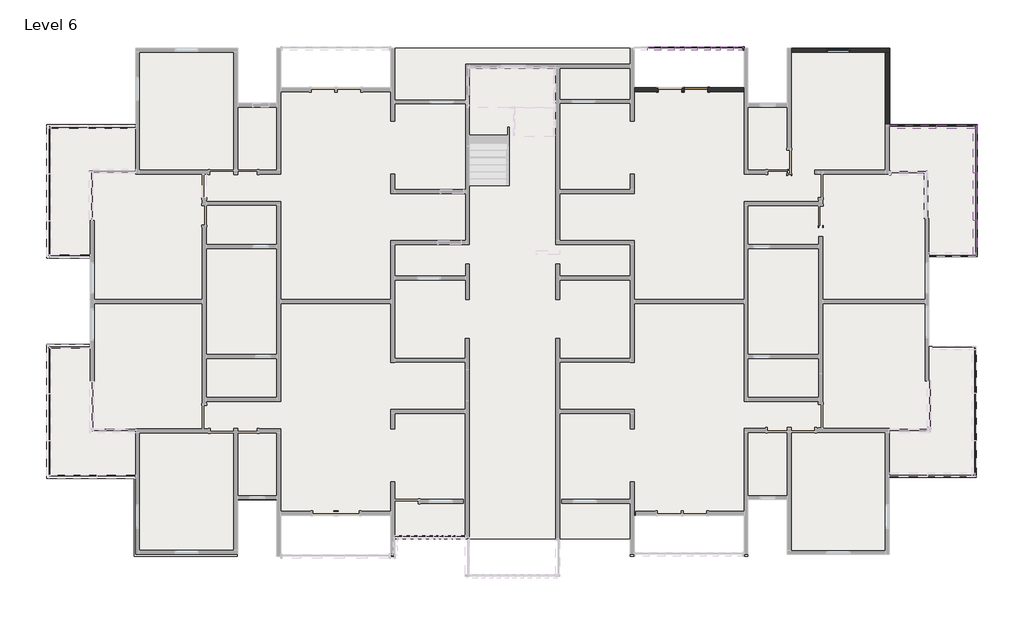
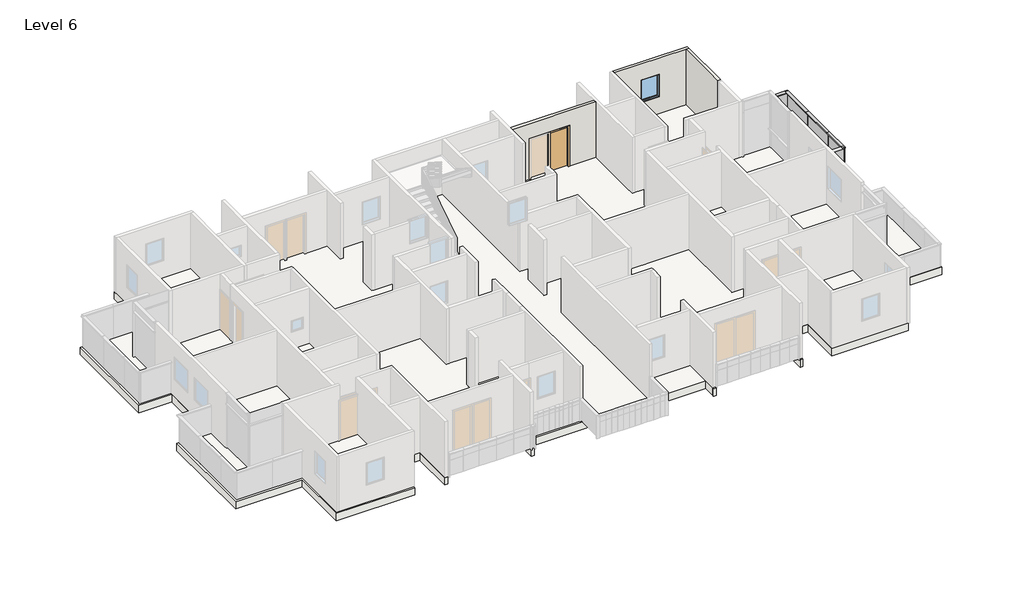
# One storey, part 5 of 7: 14 members, 13 plates, 3 walls, 1 door, 1 slab, 1 window.
"""IFC4 building model written with IfcOpenShell, lengths in millimetres."""

import ifcopenshell
import ifcopenshell.guid

model = None  # the IFC model being written
_history = None  # IfcOwnerHistory: only IFC2X3 demands one
_inside = {}  # id of a spatial element -> (the spatial element, [elements in it])
_under = {}  # id of a project, library or spatial element -> (it, [spatial elements below it])
_declared = {}  # id of a project -> (the project, [libraries it declares])
_typed = {}  # id of a type object -> (the type object, [elements of that type])
_made_of = {}  # id of a material, layer set ... -> (it, [elements and type objects made of it])


def new_model(schema):
    """Start an empty IFC model of exactly this schema.

    Asked for "IFC4X3", IfcOpenShell would pick the latest addendum, in which some entities
    have other attributes; the version numbers below select the first issue.
    IFC2X3 requires an IfcOwnerHistory on every rooted entity: one is made here for all.
    """
    global model, _history
    if schema == "IFC4X3":
        model = ifcopenshell.file(schema_version=(4, 3, 0, 0))
    else:
        model = ifcopenshell.file(schema=schema)
    _inside.clear()
    _under.clear()
    _declared.clear()
    _typed.clear()
    _made_of.clear()
    _history = None
    if model.schema == "IFC2X3":
        org = make("IfcOrganization", Name="unknown")
        user = make(
            "IfcPersonAndOrganization",
            ThePerson=make("IfcPerson", FamilyName="unknown"),
            TheOrganization=org,
        )
        app = make(
            "IfcApplication",
            ApplicationDeveloper=org,
            Version="unknown",
            ApplicationFullName="unknown",
            ApplicationIdentifier="unknown",
        )
        _history = make(
            "IfcOwnerHistory",
            OwningUser=user,
            OwningApplication=app,
            ChangeAction="ADDED",
            CreationDate=0,
        )
    return model


def make(cls, **values):
    """One entity of the class cls with the attributes given. An attribute that is None is left unset."""
    return model.create_entity(
        cls, **{name: value for name, value in values.items() if value is not None}
    )


def rooted(cls, **values):
    """An entity with a GlobalId (a new one), such as an element, a storey or a relation."""
    return make(cls, GlobalId=ifcopenshell.guid.new(), OwnerHistory=_history, **values)


def si_unit(unit_type, name, prefix=None):
    """IfcSIUnit, for example si_unit("LENGTHUNIT", "METRE", prefix="MILLI")."""
    return make("IfcSIUnit", UnitType=unit_type, Prefix=prefix, Name=name)


def assignment(units):
    """IfcUnitAssignment: the units of a project."""
    return None if units is None else make("IfcUnitAssignment", Units=units)


def point(xyz):
    """IfcCartesianPoint."""
    return None if xyz is None else make("IfcCartesianPoint", Coordinates=xyz)


def direction(xyz):
    """IfcDirection."""
    return None if xyz is None else make("IfcDirection", DirectionRatios=xyz)


def frame(location, z_axis=None, x_axis=None):
    """IfcAxis2Placement3D, a coordinate frame: its origin and axes. An axis left out is left unset."""
    return make(
        "IfcAxis2Placement3D",
        Location=point(location),
        Axis=direction(z_axis),
        RefDirection=direction(x_axis),
    )


def origin():
    """The frame at (0, 0, 0) with its axes left unset."""
    return frame((0.0, 0.0, 0.0))


def origin_with_axes():
    """The frame at (0, 0, 0) with the z axis (0, 0, 1) and the x axis (1, 0, 0) written out."""
    return frame((0.0, 0.0, 0.0), z_axis=(0.0, 0.0, 1.0), x_axis=(1.0, 0.0, 0.0))


def place(relative_to, where):
    """IfcLocalPlacement: puts the frame where relative to a parent placement (None: the world)."""
    return make(
        "IfcLocalPlacement", PlacementRelTo=relative_to, RelativePlacement=where
    )


def context(
    kind, dimensions, precision=None, world=None, true_north=None, identifier=None
):
    """IfcGeometricRepresentationContext, for example the 3D "Model" context."""
    return make(
        "IfcGeometricRepresentationContext",
        ContextIdentifier=identifier,
        ContextType=kind,
        CoordinateSpaceDimension=dimensions,
        Precision=precision,
        WorldCoordinateSystem=world,
        TrueNorth=true_north,
    )


def project(units=None, contexts=None):
    """IfcProject with its units and contexts."""
    return rooted(
        "IfcProject",
        Name="project",
        RepresentationContexts=contexts,
        UnitsInContext=assignment(units),
    )


def spatial(cls, under=None, at=None, **own):
    """A site, building, storey or space (cls), placed at a placement, below another one or the project."""
    s = rooted(cls, ObjectPlacement=at, **own)
    if under is not None:
        _under.setdefault(under.id(), (under, []))[1].append(s)
    return s


def polyline(points):
    """IfcPolyline through the points."""
    return make("IfcPolyline", Points=[point(p) for p in points])


def outline(outer, holes=None, kind="AREA"):
    """IfcArbitraryClosedProfileDef: a profile drawn as a closed curve; with holes, ...WithVoids."""
    if holes is None:
        return make("IfcArbitraryClosedProfileDef", ProfileType=kind, OuterCurve=outer)
    return make(
        "IfcArbitraryProfileDefWithVoids",
        ProfileType=kind,
        OuterCurve=outer,
        InnerCurves=holes,
    )


def extrude(swept, where, along, depth):
    """IfcExtrudedAreaSolid: the profile swept, set in the frame where, extruded along a direction by depth."""
    return make(
        "IfcExtrudedAreaSolid",
        SweptArea=swept,
        Position=where,
        ExtrudedDirection=direction(along),
        Depth=depth,
    )


def faces_of(points, faces, orient=None, outer=None):
    """IfcFace entities. A face is a list of loops; a loop is a list of indices into points, from 0.

    orient and outer hold one flag for each loop. By default every Orientation is true, the
    first loop of a face is its IfcFaceOuterBound and the others are IfcFaceBound.
    """
    made = []
    for i, loops in enumerate(faces):
        bounds = []
        for j, loop in enumerate(loops):
            is_outer = j == 0 if outer is None else outer[i][j]
            bounds.append(
                make(
                    "IfcFaceOuterBound" if is_outer else "IfcFaceBound",
                    Bound=make("IfcPolyLoop", Polygon=[points[k] for k in loop]),
                    Orientation=True if orient is None else orient[i][j],
                )
            )
        made.append(make("IfcFace", Bounds=bounds))
    return made


def faceted_brep(points, faces, orient=None, outer=None, voids=None):
    """IfcFacetedBrep: a solid bounded by flat faces; with voids (closed shells), ...WithVoids."""
    shared = [point(p) for p in points]
    hull = make("IfcClosedShell", CfsFaces=faces_of(shared, faces, orient, outer))
    if voids is None:
        return make("IfcFacetedBrep", Outer=hull)
    return make(
        "IfcFacetedBrepWithVoids",
        Outer=hull,
        Voids=[
            make(cls, CfsFaces=faces_of(shared, fs, o, b)) for cls, fs, o, b in voids
        ],
    )


def shape(context_of_items, identifier, shape_type, items):
    """IfcShapeRepresentation: the items that make up one representation, for example the "Body"."""
    return make(
        "IfcShapeRepresentation",
        ContextOfItems=context_of_items,
        RepresentationIdentifier=identifier,
        RepresentationType=shape_type,
        Items=items,
    )


def source(mapping_origin, context_of_items, identifier, shape_type, items):
    """IfcRepresentationMap: a shape defined once, which mapped items show again and again."""
    return make(
        "IfcRepresentationMap",
        MappingOrigin=mapping_origin,
        MappedRepresentation=shape(context_of_items, identifier, shape_type, items),
    )


def transform(
    local_origin,
    x_axis=None,
    y_axis=None,
    z_axis=None,
    scale=None,
    scale2=None,
    scale3=None,
    uniform=True,
):
    """IfcCartesianTransformationOperator3D, or its non-uniform kind. x_axis, y_axis, z_axis: its Axis1, 2, 3."""
    if uniform:
        return make(
            "IfcCartesianTransformationOperator3D",
            Axis1=direction(x_axis),
            Axis2=direction(y_axis),
            LocalOrigin=point(local_origin),
            Scale=scale,
            Axis3=direction(z_axis),
        )
    return make(
        "IfcCartesianTransformationOperator3DnonUniform",
        Axis1=direction(x_axis),
        Axis2=direction(y_axis),
        LocalOrigin=point(local_origin),
        Scale=scale,
        Axis3=direction(z_axis),
        Scale2=scale2,
        Scale3=scale3,
    )


def mapped(mapping_source, mapping_target):
    """IfcMappedItem: shows the shape of a source again, moved by a transform."""
    return make(
        "IfcMappedItem", MappingSource=mapping_source, MappingTarget=mapping_target
    )


def made_of(thing, what):
    """Note that an element or type object is made of a material, layer set ...; save() writes the relation."""
    if what is not None:
        _made_of.setdefault(what.id(), (what, []))[1].append(thing)
    return thing


def element(
    cls,
    number,
    at=None,
    inside=None,
    cuts=None,
    type_object=None,
    material=None,
    context=None,
    identifier="Body",
    shape_type=None,
    held_by="IfcProductDefinitionShape",
    body=None,
    shapes=None,
    **own,
):
    """One element of the class cls, such as IfcWall. Its Tag is "e" and its number.

    at: its placement. inside: the storey or other place that contains it. cuts: it is an
    opening in that element (IfcRelVoidsElement). A single representation is given by context,
    identifier, shape_type and body (its items); several are given by shapes. held_by: the class
    of the entity that holds the representations. save() writes the other relations.
    """
    e = rooted(cls, Tag="e%d" % number, ObjectPlacement=at, **own)
    if body is not None:
        shapes = [shape(context, identifier, shape_type, body)]
    if shapes is not None:
        e.Representation = make(held_by, Representations=shapes)
    if inside is not None:
        _inside.setdefault(inside.id(), (inside, []))[1].append(e)
    if cuts is not None:
        rooted(
            "IfcRelVoidsElement", RelatingBuildingElement=cuts, RelatedOpeningElement=e
        )
    if type_object is not None:
        _typed.setdefault(type_object.id(), (type_object, []))[1].append(e)
    return made_of(e, material)


def aggregate(whole, parts):
    """IfcRelAggregates: a whole, such as a stair, and the parts it consists of."""
    return rooted("IfcRelAggregates", RelatingObject=whole, RelatedObjects=parts)


def save(model, path):
    """Write the relations noted so far, then the file.

    IfcRelAggregates (storeys below a building ...), IfcRelContainedInSpatialStructure (elements
    in a storey), IfcRelDefinesByType, IfcRelAssociatesMaterial and IfcRelDeclares: one each for
    every whole, place, type object, material and project.
    """
    for whole, parts in _under.values():
        aggregate(whole, parts)
    for where, things in _inside.values():
        rooted(
            "IfcRelContainedInSpatialStructure",
            RelatedElements=things,
            RelatingStructure=where,
        )
    for kind, things in _typed.values():
        rooted("IfcRelDefinesByType", RelatedObjects=things, RelatingType=kind)
    for what, things in _made_of.values():
        rooted("IfcRelAssociatesMaterial", RelatedObjects=things, RelatingMaterial=what)
    for by, libraries in _declared.values():
        rooted("IfcRelDeclares", RelatingContext=by, RelatedDefinitions=libraries)
    model.write(path)


def m_single_flush_0915_x_2134mm_138fd904(model_context):
    return source(origin(), model_context, "Body", "SweptSolid", [
        extrude(outline(polyline([(2210.0, -533.5), (0.0, -533.5), (0.0, -457.5), (2134.0, -457.5), (2134.0, 457.5), (0.0, 457.5), (0.0, 533.5), (2210.0, 533.5), (2210.0, -533.5)])), frame((0.0, 75.0, 0.0), z_axis=(0.0, 1.0, 0.0), x_axis=(0.0, 0.0, 1.0)), (0.0, 0.0, 1.0), 25.0),
        extrude(outline(polyline([(2210.0, 533.5), (2210.0, -533.5), (0.0, -533.5), (0.0, -457.5), (2134.0, -457.5), (2134.0, 457.5), (0.0, 457.5), (0.0, 533.5), (2210.0, 533.5)])), frame((0.0, -100.0, 0.0), z_axis=(0.0, 1.0, 0.0), x_axis=(0.0, 0.0, 1.0)), (0.0, 0.0, 1.0), 25.0),
        extrude(outline(polyline([(457.5, 24.0), (-457.5, 24.0), (-457.5, 75.0), (457.5, 75.0), (457.5, 24.0)])), origin_with_axes(), (0.0, 0.0, 1.0), 2134.0),
    ])


def rectangular_mullion_50mm_x_150mm_42770ee2(model_context):
    return source(origin(), model_context, "Body", "SweptSolid", [
        extrude(outline(polyline([(0.0, 75.0), (0.0, -75.0), (-50.0, -75.0), (-50.0, 75.0), (0.0, 75.0)])), frame((0.0, 0.0, -1830.0000003), z_axis=(0.0, 0.0, 1.0), x_axis=(1.0, 0.0, 0.0)), (0.0, 0.0, 1.0), 1830.0000003),
    ])


def rectangular_mullion_50mm_x_150mm_aaee7d48(model_context):
    return source(origin(), model_context, "Body", "SweptSolid", [
        extrude(outline(polyline([(0.0, 75.0), (0.0, -75.0), (-50.0, -75.0), (-50.0, 75.0), (0.0, 75.0)])), frame((0.0, 0.0, -1830.0), z_axis=(0.0, 0.0, 1.0), x_axis=(1.0, 0.0, 0.0)), (0.0, 0.0, 1.0), 1830.0),
    ])


def rectangular_mullion_50mm_x_150mm_efa02866(model_context):
    return source(origin(), model_context, "Body", "SweptSolid", [
        extrude(outline(polyline([(0.0, 75.0), (0.0, -75.0), (-50.0, -75.0), (-50.0, 75.0), (0.0, 75.0)])), frame((0.0, 0.0, -1399.9999997), z_axis=(0.0, 0.0, 1.0), x_axis=(1.0, 0.0, 0.0)), (0.0, 0.0, 1.0), 1399.9999997),
    ])


def rectangular_mullion_50mm_x_150mm_d9f1e9e9(model_context):
    return source(origin(), model_context, "Body", "SweptSolid", [
        extrude(outline(polyline([(0.0, 75.0), (0.0, -75.0), (-50.0, -75.0), (-50.0, 75.0), (0.0, 75.0)])), frame((0.0, 0.0, -1565.8160321), z_axis=(0.0, 0.0, 1.0), x_axis=(1.0, 0.0, 0.0)), (0.0, 0.0, 1.0), 1565.8160321),
    ])


def rectangular_mullion_50mm_x_150mm_729c0cfc(model_context):
    return source(origin(), model_context, "Body", "SweptSolid", [
        extrude(outline(polyline([(0.0, 75.0), (0.0, -75.0), (-50.0, -75.0), (-50.0, 75.0), (0.0, 75.0)])), frame((0.0, 0.0, -1250.0), z_axis=(0.0, 0.0, 1.0), x_axis=(1.0, 0.0, 0.0)), (0.0, 0.0, 1.0), 1250.0),
    ])


def rectangular_mullion_50mm_x_150mm_b3666dbd(model_context):
    return source(origin(), model_context, "Body", "SweptSolid", [
        extrude(outline(polyline([(0.0, 75.0), (0.0, -75.0), (-50.0, -75.0), (-50.0, 75.0), (0.0, 75.0)])), frame((0.0, 0.0, -500.0), z_axis=(0.0, 0.0, 1.0), x_axis=(1.0, 0.0, 0.0)), (0.0, 0.0, 1.0), 500.0),
    ])


def rectangular_mullion_50mm_x_150mm_e851a0b8(model_context):
    return source(origin(), model_context, "Body", "SweptSolid", [
        extrude(outline(polyline([(0.0, 75.0), (0.0, -75.0), (-50.0, -75.0), (-50.0, 75.0), (0.0, 75.0)])), frame((0.0, 0.0, -522.7272727), z_axis=(0.0, 0.0, 1.0), x_axis=(1.0, 0.0, 0.0)), (0.0, 0.0, 1.0), 522.7272727),
    ])


def rectangular_mullion_50mm_x_150mm_e11a3e7b(model_context):
    return source(origin(), model_context, "Body", "SweptSolid", [
        extrude(outline(polyline([(0.0, 75.0), (0.0, -75.0), (-50.0, -75.0), (-50.0, 75.0), (0.0, 75.0)])), frame((0.0, 0.0, -400.0), z_axis=(0.0, 0.0, 1.0), x_axis=(1.0, 0.0, 0.0)), (0.0, 0.0, 1.0), 400.0),
    ])


def rectangular_mullion_50mm_x_150mm_23485ade(model_context):
    return source(origin(), model_context, "Body", "SweptSolid", [
        extrude(outline(polyline([(0.0, 75.0), (0.0, -75.0), (-50.0, -75.0), (-50.0, 75.0), (0.0, 75.0)])), frame((0.0, 0.0, -350.0), z_axis=(0.0, 0.0, 1.0), x_axis=(1.0, 0.0, 0.0)), (0.0, 0.0, 1.0), 350.0),
    ])


def system_panel_glazed_09fbcc53(model_context):
    return source(origin(), model_context, "Body", "SweptSolid", [
        extrude(outline(polyline([(915.0000002, 24.5), (-915.0000002, 24.5), (-915.0000002, 49.5), (915.0000002, 49.5), (915.0000002, 24.5)])), origin_with_axes(), (0.0, 0.0, 1.0), 1200.0),
    ])


def system_panel_glazed_f4bbd109(model_context):
    return source(origin(), model_context, "Body", "SweptSolid", [
        extrude(outline(polyline([(910.8343113, 24.5), (-910.8343113, 24.5), (-910.8343113, 49.5), (910.8343113, 49.5), (910.8343113, 24.5)])), origin_with_axes(), (0.0, 0.0, 1.0), 1200.0),
    ])


def system_panel_glazed_42eec186(model_context):
    return source(origin(), model_context, "Body", "SweptSolid", [
        extrude(outline(polyline([(699.9999998, 24.5), (-699.9999998, 24.5), (-699.9999998, 49.5), (699.9999998, 49.5), (699.9999998, 24.5)])), origin_with_axes(), (0.0, 0.0, 1.0), 1200.0),
    ])


def system_panel_glazed_f2fc581d(model_context):
    return source(origin(), model_context, "Body", "SweptSolid", [
        extrude(outline(polyline([(782.9080161, 24.5), (-782.9080161, 24.5), (-782.9080161, 49.5), (782.9080161, 49.5), (782.9080161, 24.5)])), origin_with_axes(), (0.0, 0.0, 1.0), 1200.0),
    ])


def system_panel_glazed_346501af(model_context):
    return source(origin(), model_context, "Body", "SweptSolid", [
        extrude(outline(polyline([(250.0, 24.5), (-250.0, 24.5), (-250.0, 49.5), (250.0, 49.5), (250.0, 24.5)])), origin_with_axes(), (0.0, 0.0, 1.0), 1200.0),
    ])


def system_panel_glazed_5241e6d5(model_context):
    return source(origin(), model_context, "Body", "SweptSolid", [
        extrude(outline(polyline([(261.3636364, 24.5), (-261.3636364, 24.5), (-261.3636364, 49.5), (261.3636364, 49.5), (261.3636364, 24.5)])), origin_with_axes(), (0.0, 0.0, 1.0), 1200.0),
    ])


def system_panel_glazed_3e660766(model_context):
    return source(origin(), model_context, "Body", "SweptSolid", [
        extrude(outline(polyline([(200.0, 24.5), (-200.0, 24.5), (-200.0, 49.5), (200.0, 49.5), (200.0, 24.5)])), origin_with_axes(), (0.0, 0.0, 1.0), 1200.0),
    ])


def system_panel_glazed_b0a6d7cd(model_context):
    return source(origin(), model_context, "Body", "SweptSolid", [
        extrude(outline(polyline([(175.0, 24.5), (-175.0, 24.5), (-175.0, 49.5), (175.0, 49.5), (175.0, 24.5)])), origin_with_axes(), (0.0, 0.0, 1.0), 1200.0),
    ])


def m_fixed_0915_x_1220mm_873aa0e2(model_context):
    return source(origin(), model_context, "Body", "SweptSolid", [
        extrude(outline(polyline([(-394.5, 53.0), (394.5, 53.0), (394.5, 41.0), (-394.5, 41.0), (-394.5, 53.0)])), frame((0.0, 0.0, 978.0), z_axis=(0.0, 0.0, 1.0), x_axis=(1.0, 0.0, 0.0)), (0.0, 0.0, 1.0), 1094.0),
        extrude(outline(polyline([(2116.0, -438.5), (934.0, -438.5), (934.0, 438.5), (2116.0, 438.5), (2116.0, -438.5)]), holes=[polyline([(2072.0, -394.5), (2072.0, 394.5), (978.0, 394.5), (978.0, -394.5), (2072.0, -394.5)])]), frame((0.0, 25.0, 0.0), z_axis=(0.0, 1.0, 0.0), x_axis=(0.0, 0.0, 1.0)), (0.0, 0.0, 1.0), 44.0),
        extrude(outline(polyline([(2135.0, -457.5), (915.0, -457.5), (915.0, 457.5), (2135.0, 457.5), (2135.0, -457.5)]), holes=[polyline([(2116.0, -438.5), (2116.0, 438.5), (934.0, 438.5), (934.0, -438.5), (2116.0, -438.5)])]), frame((0.0, 25.0, 0.0), z_axis=(0.0, 1.0, 0.0), x_axis=(0.0, 0.0, 1.0)), (0.0, 0.0, 1.0), 63.0),
        extrude(outline(polyline([(2135.0, -457.5), (915.0, -457.5), (915.0, 457.5), (2135.0, 457.5), (2135.0, -457.5)]), holes=[polyline([(2103.0, -425.5), (2103.0, 425.5), (947.0, 425.5), (947.0, -425.5), (2103.0, -425.5)])]), frame((0.0, -62.0, 0.0), z_axis=(0.0, 1.0, 0.0), x_axis=(0.0, 0.0, 1.0)), (0.0, 0.0, 1.0), 87.0),
    ])


model = new_model("IFC4")

# Units and contexts
model_context = context("Model", 3, world=origin())
ifc_project = project(units=[si_unit("LENGTHUNIT", "METRE", prefix="MILLI")], contexts=[model_context])

# Site, building, storey
site = spatial("IfcSite", under=ifc_project)
building = spatial("IfcBuilding", under=site)
storey = spatial("IfcBuildingStorey", under=building, Name="Level 6", Elevation=15500.0)

# Door
placement = place(None, origin())
m_single_flush_0915_x_2134mm_shape = m_single_flush_0915_x_2134mm_138fd904(model_context)
element("IfcDoor", 1, ObjectType="M_Single-Flush : 0915 x 2134mm", at=placement, inside=storey, context=model_context, shape_type="MappedRepresentation", body=[
    mapped(m_single_flush_0915_x_2134mm_shape, transform((6794.6515415, 8016.5690894, 15500.0), x_axis=(1.0, 0.0, 0.0), y_axis=(0.0, 1.0, 0.0), z_axis=(0.0, 0.0, 1.0))),
])

# Members
rectangular_mullion_50mm_x_150mm_shape = rectangular_mullion_50mm_x_150mm_42770ee2(model_context)
element("IfcMember", 2, ObjectType="Rectangular Mullion : 50mm x 150mm", at=placement, inside=storey, context=model_context, shape_type="MappedRepresentation", body=[
    mapped(rectangular_mullion_50mm_x_150mm_shape, transform((17635.0130284, 4788.3418163, 16750.0), x_axis=(0.0, 0.0, 1.0), y_axis=(-1.0, 0.0, 0.0), z_axis=(0.0, -1.0, 0.0))),
])
element("IfcMember", 3, ObjectType="Rectangular Mullion : 50mm x 150mm", at=placement, inside=storey, context=model_context, shape_type="MappedRepresentation", body=[
    mapped(rectangular_mullion_50mm_x_150mm_shape, transform((16129.1969963, 6568.8418166, 16750.0), x_axis=(0.0, 0.0, 1.0), y_axis=(0.0, -1.0, 0.0), z_axis=(1.0, 0.0, 0.0))),
])
rectangular_mullion_50mm_x_150mm_2_shape = rectangular_mullion_50mm_x_150mm_aaee7d48(model_context)
element("IfcMember", 4, ObjectType="Rectangular Mullion : 50mm x 150mm", at=placement, inside=storey, context=model_context, shape_type="MappedRepresentation", body=[
    mapped(rectangular_mullion_50mm_x_150mm_2_shape, transform((17635.0130284, 2958.3418163, 16750.0), x_axis=(0.0, 0.0, 1.0), y_axis=(-1.0, 0.0, 0.0), z_axis=(0.0, -1.0, 0.0))),
])
rectangular_mullion_50mm_x_150mm_3_shape = rectangular_mullion_50mm_x_150mm_efa02866(model_context)
element("IfcMember", 5, ObjectType="Rectangular Mullion : 50mm x 150mm", at=placement, inside=storey, context=model_context, shape_type="MappedRepresentation", body=[
    mapped(rectangular_mullion_50mm_x_150mm_3_shape, transform((17635.0130284, 1558.3418166, 16750.0), x_axis=(0.0, 0.0, 1.0), y_axis=(-1.0, 0.0, 0.0), z_axis=(0.0, -1.0, 0.0))),
])
rectangular_mullion_50mm_x_150mm_4_shape = rectangular_mullion_50mm_x_150mm_d9f1e9e9(model_context)
element("IfcMember", 6, ObjectType="Rectangular Mullion : 50mm x 150mm", at=placement, inside=storey, context=model_context, shape_type="MappedRepresentation", body=[
    mapped(rectangular_mullion_50mm_x_150mm_4_shape, transform((17695.0130284, 6568.8418166, 16750.0), x_axis=(0.0, 0.0, 1.0), y_axis=(0.0, -1.0, 0.0), z_axis=(1.0, 0.0, 0.0))),
])
rectangular_mullion_50mm_x_150mm_5_shape = rectangular_mullion_50mm_x_150mm_729c0cfc(model_context)
element("IfcMember", 7, ObjectType="Rectangular Mullion : 50mm x 150mm", at=placement, inside=storey, context=model_context, shape_type="MappedRepresentation", body=[
    mapped(rectangular_mullion_50mm_x_150mm_5_shape, transform((8667.3788142, 9614.2963621, 15500.0), x_axis=(1.0, 0.0, 0.0), y_axis=(0.0, -1.0, 0.0), z_axis=(0.0, 0.0, -1.0))),
])
rectangular_mullion_50mm_x_150mm_6_shape = rectangular_mullion_50mm_x_150mm_b3666dbd(model_context)
element("IfcMember", 8, ObjectType="Rectangular Mullion : 50mm x 150mm", at=placement, inside=storey, context=model_context, shape_type="MappedRepresentation", body=[
    mapped(rectangular_mullion_50mm_x_150mm_6_shape, transform((6867.3788142, 9614.2963621, 16750.0), x_axis=(0.0, 0.0, 1.0), y_axis=(0.0, -1.0, 0.0), z_axis=(1.0, 0.0, 0.0))),
])
element("IfcMember", 9, ObjectType="Rectangular Mullion : 50mm x 150mm", at=placement, inside=storey, context=model_context, shape_type="MappedRepresentation", body=[
    mapped(rectangular_mullion_50mm_x_150mm_6_shape, transform((7367.3788142, 9614.2963621, 16750.0), x_axis=(0.0, 0.0, 1.0), y_axis=(0.0, -1.0, 0.0), z_axis=(1.0, 0.0, 0.0))),
])
element("IfcMember", 10, ObjectType="Rectangular Mullion : 50mm x 150mm", at=placement, inside=storey, context=model_context, shape_type="MappedRepresentation", body=[
    mapped(rectangular_mullion_50mm_x_150mm_6_shape, transform((8267.3788142, 9614.2963621, 16750.0), x_axis=(0.0, 0.0, 1.0), y_axis=(0.0, -1.0, 0.0), z_axis=(1.0, 0.0, 0.0))),
])
rectangular_mullion_50mm_x_150mm_7_shape = rectangular_mullion_50mm_x_150mm_e851a0b8(model_context)
element("IfcMember", 11, ObjectType="Rectangular Mullion : 50mm x 150mm", at=placement, inside=storey, context=model_context, shape_type="MappedRepresentation", body=[
    mapped(rectangular_mullion_50mm_x_150mm_7_shape, transform((5444.6515415, 9614.2963621, 16750.0), x_axis=(0.0, 0.0, 1.0), y_axis=(0.0, -1.0, 0.0), z_axis=(1.0, 0.0, 0.0))),
])
element("IfcMember", 12, ObjectType="Rectangular Mullion : 50mm x 150mm", at=placement, inside=storey, context=model_context, shape_type="MappedRepresentation", body=[
    mapped(rectangular_mullion_50mm_x_150mm_7_shape, transform((5967.3788142, 9614.2963621, 16750.0), x_axis=(0.0, 0.0, 1.0), y_axis=(0.0, -1.0, 0.0), z_axis=(1.0, 0.0, 0.0))),
])
rectangular_mullion_50mm_x_150mm_8_shape = rectangular_mullion_50mm_x_150mm_e11a3e7b(model_context)
element("IfcMember", 13, ObjectType="Rectangular Mullion : 50mm x 150mm", at=placement, inside=storey, context=model_context, shape_type="MappedRepresentation", body=[
    mapped(rectangular_mullion_50mm_x_150mm_8_shape, transform((6367.3788142, 9614.2963621, 16750.0), x_axis=(0.0, 0.0, 1.0), y_axis=(0.0, -1.0, 0.0), z_axis=(1.0, 0.0, 0.0))),
])
element("IfcMember", 14, ObjectType="Rectangular Mullion : 50mm x 150mm", at=placement, inside=storey, context=model_context, shape_type="MappedRepresentation", body=[
    mapped(rectangular_mullion_50mm_x_150mm_8_shape, transform((7767.3788142, 9614.2963621, 16750.0), x_axis=(0.0, 0.0, 1.0), y_axis=(0.0, -1.0, 0.0), z_axis=(1.0, 0.0, 0.0))),
])
rectangular_mullion_50mm_x_150mm_9_shape = rectangular_mullion_50mm_x_150mm_23485ade(model_context)
element("IfcMember", 15, ObjectType="Rectangular Mullion : 50mm x 150mm", at=placement, inside=storey, context=model_context, shape_type="MappedRepresentation", body=[
    mapped(rectangular_mullion_50mm_x_150mm_9_shape, transform((8617.3788142, 9614.2963621, 16750.0), x_axis=(0.0, 0.0, 1.0), y_axis=(0.0, -1.0, 0.0), z_axis=(1.0, 0.0, 0.0))),
])

# Plates
system_panel_glazed_shape = system_panel_glazed_09fbcc53(model_context)
element("IfcPlate", 16, ObjectType="System Panel : Glazed", at=placement, inside=storey, context=model_context, shape_type="MappedRepresentation", body=[
    mapped(system_panel_glazed_shape, transform((17635.0130284, 5703.3418165, 15500.0), x_axis=(0.0, -1.0, 0.0), y_axis=(1.0, 0.0, 0.0), z_axis=(0.0, 0.0, 1.0))),
])
element("IfcPlate", 17, ObjectType="System Panel : Glazed", at=placement, inside=storey, context=model_context, shape_type="MappedRepresentation", body=[
    mapped(system_panel_glazed_shape, transform((17635.0130284, 3873.3418163, 15500.0), x_axis=(0.0, -1.0, 0.0), y_axis=(1.0, 0.0, 0.0), z_axis=(0.0, 0.0, 1.0))),
])
system_panel_glazed_2_shape = system_panel_glazed_f4bbd109(model_context)
element("IfcPlate", 18, ObjectType="System Panel : Glazed", at=placement, inside=storey, context=model_context, shape_type="MappedRepresentation", body=[
    mapped(system_panel_glazed_2_shape, transform((16748.6787171, 1608.3418166, 15500.0), x_axis=(-1.0, 0.0, 0.0), y_axis=(0.0, -1.0, 0.0), z_axis=(0.0, 0.0, 1.0))),
])
system_panel_glazed_3_shape = system_panel_glazed_42eec186(model_context)
element("IfcPlate", 19, ObjectType="System Panel : Glazed", at=placement, inside=storey, context=model_context, shape_type="MappedRepresentation", body=[
    mapped(system_panel_glazed_3_shape, transform((17635.0130284, 2258.3418165, 15500.0), x_axis=(0.0, -1.0, 0.0), y_axis=(1.0, 0.0, 0.0), z_axis=(0.0, 0.0, 1.0))),
])
system_panel_glazed_4_shape = system_panel_glazed_f2fc581d(model_context)
element("IfcPlate", 20, ObjectType="System Panel : Glazed", at=placement, inside=storey, context=model_context, shape_type="MappedRepresentation", body=[
    mapped(system_panel_glazed_4_shape, transform((16912.1050124, 6568.8418166, 15500.0), x_axis=(1.0, 0.0, 0.0), y_axis=(0.0, 1.0, 0.0), z_axis=(0.0, 0.0, 1.0))),
])
system_panel_glazed_5_shape = system_panel_glazed_346501af(model_context)
element("IfcPlate", 21, ObjectType="System Panel : Glazed", at=placement, inside=storey, context=model_context, shape_type="MappedRepresentation", body=[
    mapped(system_panel_glazed_5_shape, transform((8017.3788142, 9614.2963621, 15500.0), x_axis=(1.0, 0.0, 0.0), y_axis=(0.0, 1.0, 0.0), z_axis=(0.0, 0.0, 1.0))),
])
element("IfcPlate", 22, ObjectType="System Panel : Glazed", at=placement, inside=storey, context=model_context, shape_type="MappedRepresentation", body=[
    mapped(system_panel_glazed_5_shape, transform((7117.3788142, 9614.2963621, 15500.0), x_axis=(1.0, 0.0, 0.0), y_axis=(0.0, 1.0, 0.0), z_axis=(0.0, 0.0, 1.0))),
])
element("IfcPlate", 23, ObjectType="System Panel : Glazed", at=placement, inside=storey, context=model_context, shape_type="MappedRepresentation", body=[
    mapped(system_panel_glazed_5_shape, transform((6617.3788142, 9614.2963621, 15500.0), x_axis=(1.0, 0.0, 0.0), y_axis=(0.0, 1.0, 0.0), z_axis=(0.0, 0.0, 1.0))),
])
system_panel_glazed_6_shape = system_panel_glazed_5241e6d5(model_context)
element("IfcPlate", 24, ObjectType="System Panel : Glazed", at=placement, inside=storey, context=model_context, shape_type="MappedRepresentation", body=[
    mapped(system_panel_glazed_6_shape, transform((5706.0151778, 9614.2963621, 15500.0), x_axis=(1.0, 0.0, 0.0), y_axis=(0.0, 1.0, 0.0), z_axis=(0.0, 0.0, 1.0))),
])
element("IfcPlate", 25, ObjectType="System Panel : Glazed", at=placement, inside=storey, context=model_context, shape_type="MappedRepresentation", body=[
    mapped(system_panel_glazed_6_shape, transform((5183.2879051, 9614.2963621, 15500.0), x_axis=(1.0, 0.0, 0.0), y_axis=(0.0, 1.0, 0.0), z_axis=(0.0, 0.0, 1.0))),
])
system_panel_glazed_7_shape = system_panel_glazed_3e660766(model_context)
element("IfcPlate", 26, ObjectType="System Panel : Glazed", at=placement, inside=storey, context=model_context, shape_type="MappedRepresentation", body=[
    mapped(system_panel_glazed_7_shape, transform((7567.3788142, 9614.2963621, 15500.0), x_axis=(1.0, 0.0, 0.0), y_axis=(0.0, 1.0, 0.0), z_axis=(0.0, 0.0, 1.0))),
])
element("IfcPlate", 27, ObjectType="System Panel : Glazed", at=placement, inside=storey, context=model_context, shape_type="MappedRepresentation", body=[
    mapped(system_panel_glazed_7_shape, transform((6167.3788142, 9614.2963621, 15500.0), x_axis=(1.0, 0.0, 0.0), y_axis=(0.0, 1.0, 0.0), z_axis=(0.0, 0.0, 1.0))),
])
system_panel_glazed_8_shape = system_panel_glazed_b0a6d7cd(model_context)
element("IfcPlate", 28, ObjectType="System Panel : Glazed", at=placement, inside=storey, context=model_context, shape_type="MappedRepresentation", body=[
    mapped(system_panel_glazed_8_shape, transform((8442.3788142, 9614.2963621, 15500.0), x_axis=(1.0, 0.0, 0.0), y_axis=(0.0, 1.0, 0.0), z_axis=(0.0, 0.0, 1.0))),
])

# Slab
element("IfcSlab", 29, ObjectType="Generic Floor - 400mm", at=placement, inside=storey, context=model_context, shape_type="SweptSolid", body=[
    extrude(outline(polyline([(-10978.0757313, 7482.4781803), (-9455.3484585, 7482.4781803), (-9455.3484585, 9614.2963621), (-9305.3484585, 9614.2963621), (-9305.3484585, 8091.5690894), (-5039.4393676, 8091.5690894), (-5039.4393676, 9614.2963621), (4399.196996, 9614.2963621), (4399.196996, 8091.5690894), (8665.1060869, 8091.5690894), (8665.1060869, 9614.2963621), (8817.3788142, 9614.2963621), (8817.3788142, 7482.4781803), (10342.3783683, 7482.4781803), (10342.3783683, 9614.2963621), (14312.8444058, 9614.2963621), (14312.8444058, 6653.3418166), (17717.8444058, 6653.3418166), (17717.8444058, 1533.3418166), (15837.8444058, 1533.3418166), (15837.8444058, -1946.1581834), (17677.8444058, -1946.1581834), (17677.8444058, -7028.8854561), (14240.1060869, -7028.8854561), (14240.1060869, -10028.8854561), (10340.1060869, -10028.8854561), (10340.1060869, -7894.794547), (8815.1060869, -7894.794547), (8815.1060869, -10106.1581834), (8665.1060869, -10106.1581834), (8665.1060869, -8506.1581834), (4401.4697233, -8506.1581834), (4401.4697233, -10106.1581834), (4251.4697233, -10106.1581834), (4251.4697233, -10028.8854561), (4251.4697233, -9417.5218198), (-4887.1666404, -9417.5218198), (-4887.1666404, -10006.7413208), (-4887.1666404, -10106.1581834), (-5039.4393676, -10106.1581834), (-5039.4393676, -8503.8854561), (-9303.0757313, -8503.8854561), (-9303.0757313, -10106.1581834), (-9453.0757313, -10106.1581834), (-9453.0757313, -7906.1581834), (-10989.3512663, -7906.1581834), (-10989.3512663, -10106.1581834), (-14989.3512663, -10106.1581834), (-14989.3512663, -7083.4309107), (-18389.3512663, -7083.4309107), (-18389.3512663, -1883.4309107), (-16697.1666404, -1883.4309107), (-16697.1666404, 1474.2963621), (-18377.1666404, 1474.2963621), (-18377.1666404, 6654.2963621), (-14937.1666404, 6654.2963621), (-14937.1666404, 9614.2963621), (-10978.0757313, 9614.2963621), (-10978.0757313, 7482.4781803)])), frame((0.0, 0.0, 15100.0), z_axis=(0.0, 0.0, 1.0), x_axis=(1.0, 0.0, 0.0)), (0.0, 0.0, 1.0), 400.0),
])

# Walls
element("IfcWall", 30, ObjectType="wal 150", at=placement, inside=storey, context=model_context, shape_type="SweptSolid", body=[
    extrude(outline(polyline([(15500.0, 8665.1060869), (18500.0, 8665.1060869), (18500.0, 4399.196996), (15500.0, 4399.196996), (15500.0, 5337.1515415), (17634.0, 5337.1515415), (17634.0, 6252.1515415), (15500.0, 6252.1515415), (15500.0, 6337.1515415), (17634.0, 6337.1515415), (17634.0, 7252.1515415), (15500.0, 7252.1515415), (15500.0, 8665.1060869)])), frame((0.0, 7941.5690894, 0.0), z_axis=(0.0, 1.0, 0.0), x_axis=(0.0, 0.0, 1.0)), (0.0, 0.0, 1.0), 150.0),
])
element("IfcWall", 31, ObjectType="wal 150", at=placement, inside=storey, context=model_context, shape_type="Brep", body=[
    faceted_brep([(10492.3783683, 9464.2963621, 15500.0), (14149.196996, 9464.2963621, 15500.0), (14299.196996, 9464.2963621, 15500.0), (14299.196996, 9464.2963621, 18500.0), (14149.196996, 9464.2963621, 18500.0), (10492.3783683, 9464.2963621, 18500.0), (11863.2876822, 9464.2963621, 16415.0), (11863.2876822, 9464.2963621, 17635.0), (12778.2876822, 9464.2963621, 17635.0), (12778.2876822, 9464.2963621, 16415.0), (10492.3783683, 9614.2963621, 15500.0), (10492.3783683, 9614.2963621, 18500.0), (14299.196996, 9614.2963621, 18500.0), (14299.196996, 9614.2963621, 15500.0), (11863.2876822, 9614.2963621, 16415.0), (12778.2876822, 9614.2963621, 16415.0), (12778.2876822, 9614.2963621, 17635.0), (11863.2876822, 9614.2963621, 17635.0)], [[[0, 1, 2, 3, 4, 5], [6, 7, 8, 9]], [[10, 11, 12, 13], [14, 15, 16, 17]], [[2, 1, 0, 10, 13]], [[5, 4, 3, 12, 11]], [[7, 6, 14, 17]], [[8, 7, 17, 16]], [[9, 8, 16, 15]], [[6, 9, 15, 14]], [[0, 5, 11, 10]], [[3, 2, 13, 12]]]),
])
element("IfcWall", 32, ObjectType="wal 150", at=placement, inside=storey, context=model_context, shape_type="SweptSolid", body=[
    extrude(outline(polyline([(14149.196996, 6668.8418166), (14149.196996, 9464.2963621), (14299.196996, 9464.2963621), (14299.196996, 6668.8418166), (14149.196996, 6668.8418166)])), frame((0.0, 0.0, 15500.0), z_axis=(0.0, 0.0, 1.0), x_axis=(1.0, 0.0, 0.0)), (0.0, 0.0, 1.0), 3000.0),
])

# Window
m_fixed_0915_x_1220mm_shape = m_fixed_0915_x_1220mm_873aa0e2(model_context)
element("IfcWindow", 33, ObjectType="M_Fixed : 1.80 to 1.20 w2", at=placement, inside=storey, context=model_context, shape_type="MappedRepresentation", body=[
    mapped(m_fixed_0915_x_1220mm_shape, transform((12320.7876822, 9526.2963621, 15500.0), x_axis=(1.0, 0.0, 0.0), y_axis=(0.0, 1.0, 0.0), z_axis=(0.0, 0.0, 1.0))),
])

save(model, "model.ifc")

# Revit data of these elements
# Type "M_Single-Flush : 0915 x 2134mm"
#   Type Mark = "15"
#   Thickness = 0.051 m
#   Height = 2.134 m
#   Trim Projection Ext = 0.025 m
#   Trim Projection Int = 0.025 m
#   Trim Width = 0.076 m
#   Width = 0.915 m
#   Door Material = Door - Panel
#   Frame Material = Door - Frame
#   Function = (empty or 0)
#   Wall Closure = (empty or 0)
# Type "Rectangular Mullion : 50mm x 150mm"
#   built-in parameter 1007304 = 0.492126 (stored number, unit not read)
#   built-in parameter 1007301 = 0.082021 (stored number, unit not read)
#   built-in parameter 1007300 = 0.082021 (stored number, unit not read)
# Type "Generic Floor - 400mm"
#   Function = 0
#   Layers, outside or top first: 0.4 m no material (function 1)
# Type "wal 150"
#   Layers, outside or top first: 0.15 m no material (function 1)
# Type "M_Fixed : 1.80 to 1.20 w2"
#   Type Mark = "19"
#   Height = 1.22 m
#   Default Sill Height = 0.915 m
#   Width = 0.915 m
#   Window Inset = 0.019 m
#   Frame Exterior Material = Sash
#   Frame Interior Material = Sash
#   Glass Pane Material = Glass
#   Sash = Sash
#   Wall Closure = (empty or 0)
# Element 1 (IfcDoor, "M_Single-Flush : 0915 x 2134mm")
#   Phase Created = New Construction
#   Materials on its faces: "Door - Frame", "Door - Panel"
# Elements 2, 3, 4, 5, 6, 7, 8, 9, 10, 11, 12, 13, 14, 15 (IfcMember, "Rectangular Mullion : 50mm x 150mm")
#   Phase Created = New Construction
#   Materials on its faces: "Aluminum"
# Elements 16, 17, 18, 19, 20, 21, 22, 23, 24, 25, 26, 27, 28 (IfcPlate, "System Panel : Glazed")
#   Phase Created = New Construction
#   Materials on its faces: "Glass"
# Element 29 (IfcSlab, "Generic Floor - 400mm")
#   built-in parameter 1001955 = 3.14159 (stored number, unit not read)
#   Height Offset From Level = 0 m
#   Phase Created = New Construction
#   Materials on its faces: "Default Roof", "Door - Frame", "Ceiling Tile 600 x 1200", "Oak Flooring"
# Element 30 (IfcWall, "wal 150")
#   Top Offset = 0 m
#   Base Offset = 0 m
#   Unconnected Height = 3 m
#   wall height = 3 m
#   Phase Created = New Construction
#   Base Constraint = Level 6
#   Materials on its faces: "Default Wall", "Door - Frame"
# Element 31 (IfcWall, "wal 150")
#   Top Offset = 0 m
#   Base Offset = 0 m
#   Unconnected Height = 3 m
#   wall height = 3 m
#   Phase Created = New Construction
#   Base Constraint = Level 6
#   Materials on its faces: "Default Wall", "Ceiling Tile 600 x 600", "Ceiling Tile 600 x 1200"
# Element 32 (IfcWall, "wal 150")
#   Top Offset = 0 m
#   Base Offset = 0 m
#   Unconnected Height = 3 m
#   wall height = 3 m
#   Phase Created = New Construction
#   Base Constraint = Level 6
#   Materials on its faces: "Default Wall", "Ceiling Tile 600 x 1200"
# Element 33 (IfcWindow, "M_Fixed : 1.80 to 1.20 w2")
#   Mark = "375"
#   Phase Created = New Construction
#   Materials on its faces: "Sash", "Glass"
# Materials
#   "Door - Panel": class "Wood", colour RGB 114 82 51, transparency 0
#   "Door - Frame": class "Miscellaneous", colour RGB 255 0 128, transparency 0, Cost = 0
#   "Sash": class "Wood", colour RGB 136 99 55, transparency 0
#   "Glass": class "Glass", colour RGB 218 227 224, transparency 0.85, Description = "Soda Lime Glass", Cost = 0
#   "Aluminum": class "Metal", colour RGB 244 244 244, transparency 0, Description = "Aluminum 6061", Cost = 0
#   "Default Roof": class "Miscellaneous", colour RGB 80 80 80, transparency 0
#   "Ceiling Tile 600 x 1200": class "Generic", colour RGB 179 178 175, transparency 0, Description = "Acoustic ceiling tile", Cost = 0
#   "Oak Flooring": class "Wood", colour RGB 216 169 114, transparency 0, Description = "Quercus Rubra", Cost = 0
#   "Default Wall": class "Miscellaneous", colour RGB 80 80 80, transparency 0
#   "Ceiling Tile 600 x 600": class "Generic", colour RGB 180 179 177, transparency 0, Description = "Acoustic ceiling tile", Cost = 0
